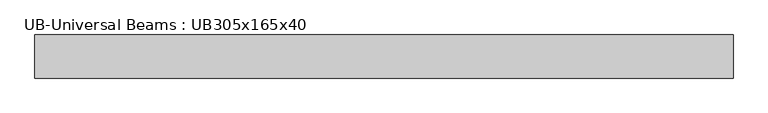
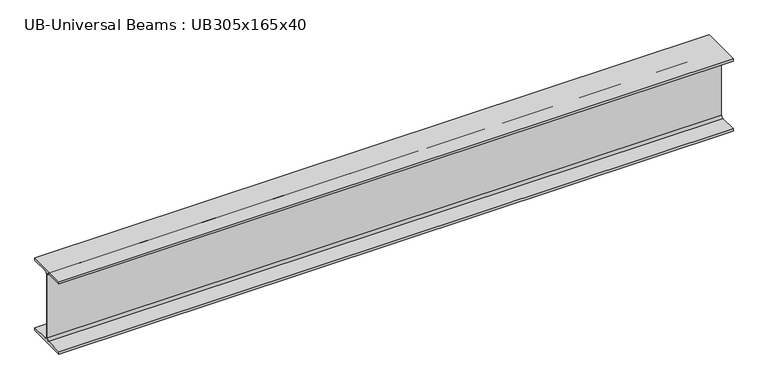
"""IFC4 building model written with IfcOpenShell, lengths in millimetres: beam geometry, UB-Universal Beams : UB305x165x40."""

from ifc_helpers import new_model, si_unit, point, frame, frame_2d, origin, place, context, project, spatial, polyline, circle_curve, trimmed, segment, composite_curve, outline, extrude, source, transform, mapped, element, save


def ub_universal_beams_ub305x165x40_8f112fac(model_context):
    return source(origin(), model_context, "Body", "SweptSolid", [
        extrude(outline(composite_curve([segment(polyline([(82.5, -141.5), (82.5, -151.7), (-82.5, -151.7), (-82.5, -141.5), (-11.9, -141.5)]), True, "CONTINUOUS"), segment(trimmed(circle_curve(frame_2d((-11.9, -132.6)), 8.9), [point((-11.9, -141.5))], [point((-3.0, -132.6))], True, "CARTESIAN"), True, "CONTINUOUS"), segment(polyline([(-3.0, -132.6), (-3.0, 132.6)]), True, "CONTINUOUS"), segment(trimmed(circle_curve(frame_2d((-11.9, 132.6)), 8.9), [point((-3.0, 132.6))], [point((-11.9, 141.5))], True, "CARTESIAN"), True, "CONTINUOUS"), segment(polyline([(-11.9, 141.5), (-82.5, 141.5), (-82.5, 151.7), (82.5, 151.7), (82.5, 141.5), (11.9, 141.5)]), True, "CONTINUOUS"), segment(trimmed(circle_curve(frame_2d((11.9, 132.6)), 8.9), [point((11.9, 141.5))], [point((3.0, 132.6))], True, "CARTESIAN"), True, "CONTINUOUS"), segment(polyline([(3.0, 132.6), (3.0, -132.6)]), True, "CONTINUOUS"), segment(trimmed(circle_curve(frame_2d((11.9, -132.6)), 8.9), [point((3.0, -132.6))], [point((11.9, -141.5))], True, "CARTESIAN"), True, "CONTINUOUS"), segment(polyline([(11.9, -141.5), (82.5, -141.5)]), True, "CONTINUOUS")], self_intersect=False)), frame((-1334.6, 0.0, 0.0), z_axis=(1.0, 0.0, 0.0), x_axis=(0.0, 1.0, 0.0)), (0.0, 0.0, 1.0), 2669.2),
    ])


if __name__ == "__main__":
    model = new_model("IFC4")
    model_context = context("Model", 3, world=origin())
    ifc_project = project(units=[si_unit("LENGTHUNIT", "METRE", prefix="MILLI")], contexts=[model_context])
    site = spatial("IfcSite", under=ifc_project)
    building = spatial("IfcBuilding", under=site)
    placement = place(None, origin())
    ub_universal_beams_ub305x165x40_shape = ub_universal_beams_ub305x165x40_8f112fac(model_context)
    element("IfcBeam", 1, ObjectType="UB-Universal Beams : UB305x165x40", at=placement, inside=building, context=model_context, shape_type="MappedRepresentation", body=[
        mapped(ub_universal_beams_ub305x165x40_shape, transform((0.0, 0.0, 0.0), x_axis=(1.0, 0.0, 0.0), y_axis=(0.0, 1.0, 0.0), z_axis=(0.0, 0.0, 1.0))),
    ])
    save(model, "model.ifc")

# Revit data of these elements
# Type "UB-Universal Beams : UB305x165x40"
#   Section Name Key = "UB305X165X40"
#   Width = 16.5 cm
#   Web Thickness = 0.6 cm
#   Web Fillet = 0.89 cm
#   Warping Constant = 164000.0 cm⁶
#   Torsional Moment of Inertia = 14.70 cm⁴
#   Section Area = 51.3 cm²
#   Plastic Modulus weak axis = 142.0 cm³
#   Plastic Modulus strong axis = 623.0 cm³
#   Nominal Weight = 40.2999 kgf/m
#   Moment of Inertia weak axis = 764.00 cm⁴
#   Moment of Inertia strong axis = 8503.00 cm⁴
#   Height = 30.34 cm
#   Flange Thickness = 1.02 cm
#   Elastic Modulus weak axis = 92.6 cm³
#   Elastic Modulus strong axis = 560.0 cm³
#   Centroid Vertical = 15.17 cm
#   Centroid Horizontal = 8.25 cm
#   Bolt Spacing = 9.0 cm
#   Length [instance default] = 1500 mm
#   Structural Material [instance default] = Metal - Steel 43-275
#   Type Comments = ""
#   Assembly Code = ""
# Element 1 (IfcBeam, "UB-Universal Beams : UB305x165x40")
#   Materials on its faces: "Metal - Steel 43-275"
# Materials
#   "Metal - Steel 43-275": class "Metal", colour RGB 247 247 247, transparency 0, Cost = 0
